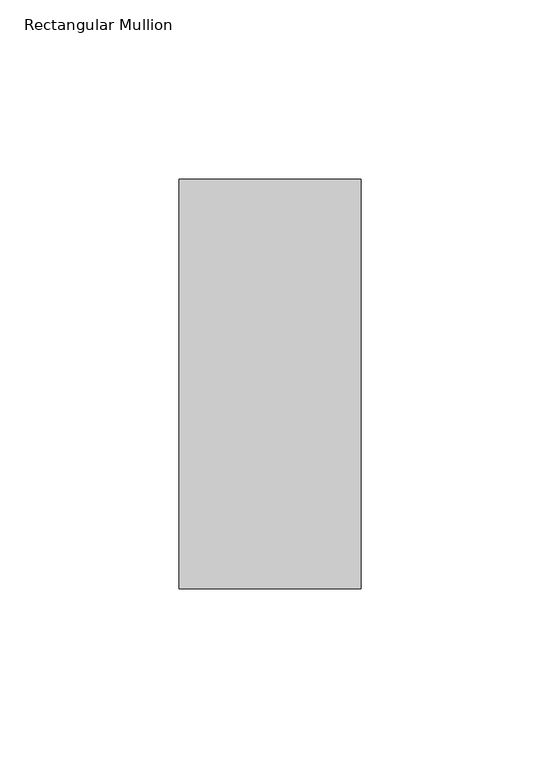
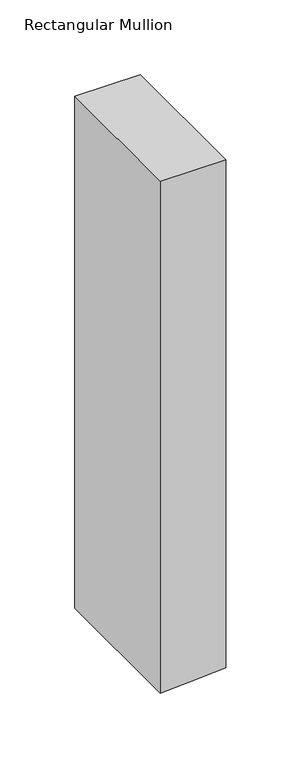
"""IFC4 building model written with IfcOpenShell, lengths in millimetres: member geometry, Rectangular Mullion : KAWNEER TRIFAB VERSAGLAZE 451T - CLEAR ANODIZED ALUM. - BACK GLAZED."""

from ifc_helpers import new_model, si_unit, frame, origin, place, context, project, spatial, polyline, outline, extrude, source, transform, mapped, element, save


def rectangular_mullion_0cc3a6c5(model_context):
    return source(origin(), model_context, "Body", "SweptSolid", [
        extrude(outline(polyline([(0.0, 25.4), (0.0, -25.4), (-418.207128, -25.4), (-416.817679, -3.1688169), (-415.032128, 25.4), (0.0, 25.4)])), frame((0.0, -57.15, 0.0), z_axis=(0.0, 1.0, 0.0), x_axis=(0.0, 0.0, 1.0)), (0.0, 0.0, 1.0), 114.3),
    ])


if __name__ == "__main__":
    model = new_model("IFC4")
    model_context = context("Model", 3, world=origin())
    ifc_project = project(units=[si_unit("LENGTHUNIT", "METRE", prefix="MILLI")], contexts=[model_context])
    site = spatial("IfcSite", under=ifc_project)
    building = spatial("IfcBuilding", under=site)
    placement = place(None, origin())
    rectangular_mullion_shape = rectangular_mullion_0cc3a6c5(model_context)
    element("IfcMember", 1, ObjectType="Rectangular Mullion : KAWNEER TRIFAB VERSAGLAZE 451T - CLEAR ANODIZED ALUM. - BACK GLAZED", at=placement, inside=building, context=model_context, shape_type="MappedRepresentation", body=[
        mapped(rectangular_mullion_shape, transform((0.0, 0.0, 0.0), x_axis=(1.0, 0.0, 0.0), y_axis=(0.0, 1.0, 0.0), z_axis=(0.0, 0.0, 1.0))),
    ])
    save(model, "model.ifc")

# Revit data of these elements
# Type "Rectangular Mullion : KAWNEER TRIFAB VERSAGLAZE 451T - CLEAR ANODIZED ALUM. - BACK GLAZED"
#   built-in parameter 1007304 = 0.375 (stored number, unit not read)
#   built-in parameter 1007301 = 0.0833333 (stored number, unit not read)
#   built-in parameter 1007300 = 0.0833333 (stored number, unit not read)
# Element 1 (IfcMember, "Rectangular Mullion : KAWNEER TRIFAB VERSAGLAZE 451T - CLEAR ANODIZED ALUM. - BACK GLAZED")
#   Materials on its faces: "KAWNEER TRIFAB VERSAGLAZE 451T - CLEAR ANODIZED ALUM. - BACK GLAZED"
# Materials
#   "KAWNEER TRIFAB VERSAGLAZE 451T - CLEAR ANODIZED ALUM. - BACK GLAZED": class "Metal", colour RGB 244 244 244, transparency 0, Description = "Aluminum 6061", Cost = 0
